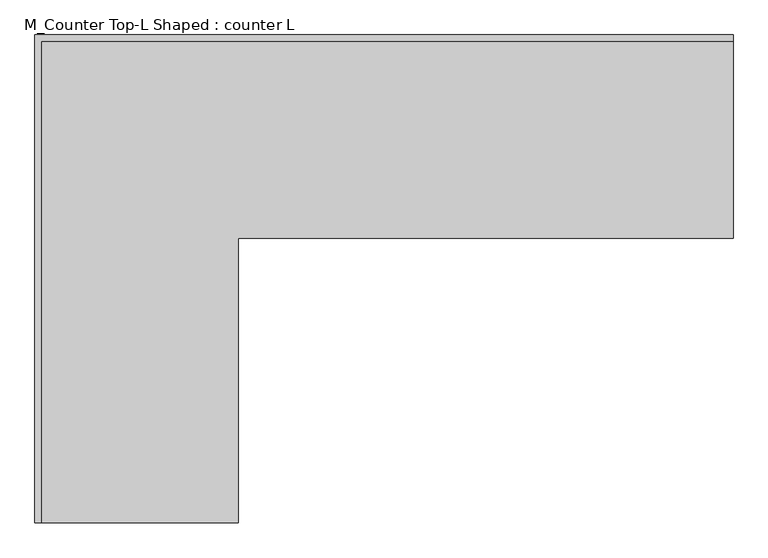
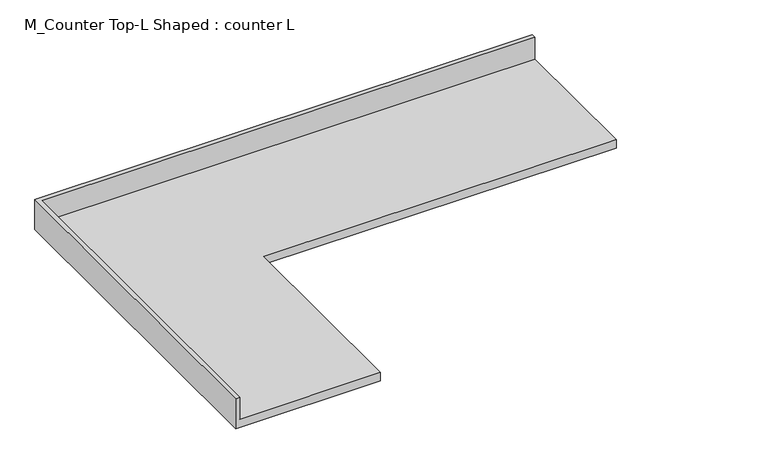
"""IFC4 building model written with IfcOpenShell, lengths in millimetres: furniture geometry, M_Counter Top-L Shaped : counter L."""

from ifc_helpers import new_model, si_unit, origin, place, context, project, spatial, faceted_brep, source, transform, mapped, element, save


def m_counter_top_l_shaped_counter_l_676b1070(model_context):
    return source(origin(), model_context, "Body", "Brep", [
        faceted_brep([(-565.4622951, -1524.0, 914.4), (-565.4622951, -635.0, 914.4), (980.8783694, -635.0, 914.4), (980.8783694, -19.05, 914.4), (-1181.4122951, -19.05, 914.4), (-1181.4122951, -1524.0, 914.4), (980.8783694, 0.0, 876.3), (980.8783694, -635.0, 876.3), (-565.4622951, -635.0, 876.3), (-565.4622951, -1524.0, 876.3), (-1200.4622951, -1524.0, 876.3), (-1200.4622951, 0.0, 876.3), (-1200.4622951, 0.0, 1016.0), (980.8783694, 0.0, 1016.0), (-1200.4622951, -1524.0, 1016.0), (-1181.4122951, -1524.0, 1016.0), (980.8783694, -19.05, 1016.0), (-1181.4122951, -19.05, 1016.0)], [[[0, 1, 2, 3, 4, 5]], [[6, 7, 8, 9, 10, 11]], [[6, 11, 12, 13]], [[11, 10, 14, 12]], [[14, 10, 9, 0, 5, 15]], [[1, 0, 9, 8]], [[2, 1, 8, 7]], [[7, 6, 13, 16, 3, 2]], [[12, 14, 15, 17, 16, 13]], [[3, 16, 17, 4]], [[17, 15, 5, 4]]]),
    ])


if __name__ == "__main__":
    model = new_model("IFC4")
    model_context = context("Model", 3, world=origin())
    ifc_project = project(units=[si_unit("LENGTHUNIT", "METRE", prefix="MILLI")], contexts=[model_context])
    site = spatial("IfcSite", under=ifc_project)
    building = spatial("IfcBuilding", under=site)
    placement = place(None, origin())
    m_counter_top_l_shaped_counter_l_shape = m_counter_top_l_shaped_counter_l_676b1070(model_context)
    element("IfcFurniture", 1, ObjectType="M_Counter Top-L Shaped : counter L", at=placement, inside=building, context=model_context, shape_type="MappedRepresentation", body=[
        mapped(m_counter_top_l_shaped_counter_l_shape, transform((0.0, 0.0, 0.0), x_axis=(1.0, 0.0, 0.0), y_axis=(0.0, 1.0, 0.0), z_axis=(0.0, 0.0, 1.0))),
    ])
    save(model, "model.ifc")

# Revit data of these elements
# Type "M_Counter Top-L Shaped : counter L"
#   Counter Thickness = 0' - 1 1/2"
#   Depth = 2' - 1"
#   Height = 3' - 0"
#   Length - Leg 1 [instance default] = 8' - 2.4252"
#   Length - Leg 2 [instance default] = 5' - 10.86614"
#   Counter Top Material = Counter Top
#   Default Elevation = 0
# Element 1 (IfcFurniture, "M_Counter Top-L Shaped : counter L")
#   Length - Leg 1 = 7' - 1.87955"
#   Length - Leg 2 = 5' - 0"
#   Materials on its faces: "Counter Top"
# Materials
#   "Counter Top": class "Wood", colour RGB 226 177 128, transparency 0
